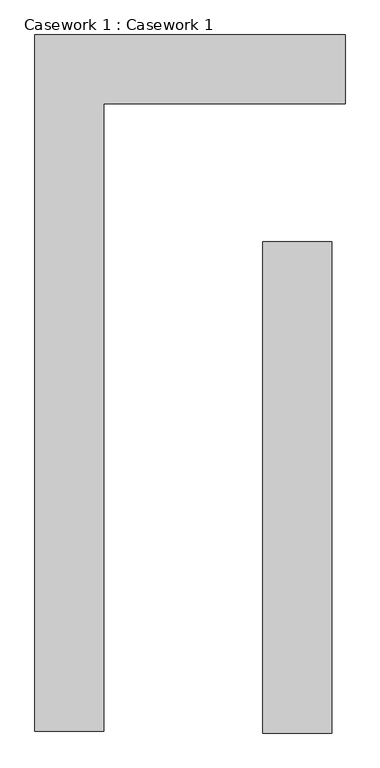
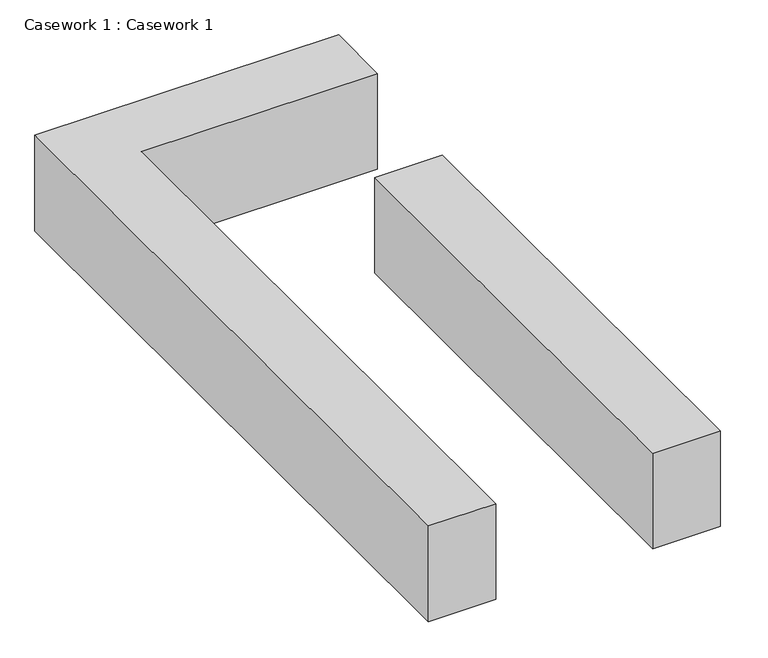
"""IFC4 building model written with IfcOpenShell, lengths in millimetres: furniture geometry, Casework 1 : Casework 1."""

import ifcopenshell
import ifcopenshell.guid

model = None  # the IFC model being written
_history = None  # IfcOwnerHistory: only IFC2X3 demands one
_inside = {}  # id of a spatial element -> (the spatial element, [elements in it])
_under = {}  # id of a project, library or spatial element -> (it, [spatial elements below it])
_declared = {}  # id of a project -> (the project, [libraries it declares])
_typed = {}  # id of a type object -> (the type object, [elements of that type])
_made_of = {}  # id of a material, layer set ... -> (it, [elements and type objects made of it])


def new_model(schema):
    """Start an empty IFC model of exactly this schema.

    Asked for "IFC4X3", IfcOpenShell would pick the latest addendum, in which some entities
    have other attributes; the version numbers below select the first issue.
    IFC2X3 requires an IfcOwnerHistory on every rooted entity: one is made here for all.
    """
    global model, _history
    if schema == "IFC4X3":
        model = ifcopenshell.file(schema_version=(4, 3, 0, 0))
    else:
        model = ifcopenshell.file(schema=schema)
    _inside.clear()
    _under.clear()
    _declared.clear()
    _typed.clear()
    _made_of.clear()
    _history = None
    if model.schema == "IFC2X3":
        org = make("IfcOrganization", Name="unknown")
        user = make(
            "IfcPersonAndOrganization",
            ThePerson=make("IfcPerson", FamilyName="unknown"),
            TheOrganization=org,
        )
        app = make(
            "IfcApplication",
            ApplicationDeveloper=org,
            Version="unknown",
            ApplicationFullName="unknown",
            ApplicationIdentifier="unknown",
        )
        _history = make(
            "IfcOwnerHistory",
            OwningUser=user,
            OwningApplication=app,
            ChangeAction="ADDED",
            CreationDate=0,
        )
    return model


def make(cls, **values):
    """One entity of the class cls with the attributes given. An attribute that is None is left unset."""
    return model.create_entity(
        cls, **{name: value for name, value in values.items() if value is not None}
    )


def rooted(cls, **values):
    """An entity with a GlobalId (a new one), such as an element, a storey or a relation."""
    return make(cls, GlobalId=ifcopenshell.guid.new(), OwnerHistory=_history, **values)


def si_unit(unit_type, name, prefix=None):
    """IfcSIUnit, for example si_unit("LENGTHUNIT", "METRE", prefix="MILLI")."""
    return make("IfcSIUnit", UnitType=unit_type, Prefix=prefix, Name=name)


def assignment(units):
    """IfcUnitAssignment: the units of a project."""
    return None if units is None else make("IfcUnitAssignment", Units=units)


def point(xyz):
    """IfcCartesianPoint."""
    return None if xyz is None else make("IfcCartesianPoint", Coordinates=xyz)


def direction(xyz):
    """IfcDirection."""
    return None if xyz is None else make("IfcDirection", DirectionRatios=xyz)


def frame(location, z_axis=None, x_axis=None):
    """IfcAxis2Placement3D, a coordinate frame: its origin and axes. An axis left out is left unset."""
    return make(
        "IfcAxis2Placement3D",
        Location=point(location),
        Axis=direction(z_axis),
        RefDirection=direction(x_axis),
    )


def origin():
    """The frame at (0, 0, 0) with its axes left unset."""
    return frame((0.0, 0.0, 0.0))


def origin_with_axes():
    """The frame at (0, 0, 0) with the z axis (0, 0, 1) and the x axis (1, 0, 0) written out."""
    return frame((0.0, 0.0, 0.0), z_axis=(0.0, 0.0, 1.0), x_axis=(1.0, 0.0, 0.0))


def place(relative_to, where):
    """IfcLocalPlacement: puts the frame where relative to a parent placement (None: the world)."""
    return make(
        "IfcLocalPlacement", PlacementRelTo=relative_to, RelativePlacement=where
    )


def context(
    kind, dimensions, precision=None, world=None, true_north=None, identifier=None
):
    """IfcGeometricRepresentationContext, for example the 3D "Model" context."""
    return make(
        "IfcGeometricRepresentationContext",
        ContextIdentifier=identifier,
        ContextType=kind,
        CoordinateSpaceDimension=dimensions,
        Precision=precision,
        WorldCoordinateSystem=world,
        TrueNorth=true_north,
    )


def project(units=None, contexts=None):
    """IfcProject with its units and contexts."""
    return rooted(
        "IfcProject",
        Name="project",
        RepresentationContexts=contexts,
        UnitsInContext=assignment(units),
    )


def spatial(cls, under=None, at=None, **own):
    """A site, building, storey or space (cls), placed at a placement, below another one or the project."""
    s = rooted(cls, ObjectPlacement=at, **own)
    if under is not None:
        _under.setdefault(under.id(), (under, []))[1].append(s)
    return s


def polyline(points):
    """IfcPolyline through the points."""
    return make("IfcPolyline", Points=[point(p) for p in points])


def outline(outer, holes=None, kind="AREA"):
    """IfcArbitraryClosedProfileDef: a profile drawn as a closed curve; with holes, ...WithVoids."""
    if holes is None:
        return make("IfcArbitraryClosedProfileDef", ProfileType=kind, OuterCurve=outer)
    return make(
        "IfcArbitraryProfileDefWithVoids",
        ProfileType=kind,
        OuterCurve=outer,
        InnerCurves=holes,
    )


def extrude(swept, where, along, depth):
    """IfcExtrudedAreaSolid: the profile swept, set in the frame where, extruded along a direction by depth."""
    return make(
        "IfcExtrudedAreaSolid",
        SweptArea=swept,
        Position=where,
        ExtrudedDirection=direction(along),
        Depth=depth,
    )


def shape(context_of_items, identifier, shape_type, items):
    """IfcShapeRepresentation: the items that make up one representation, for example the "Body"."""
    return make(
        "IfcShapeRepresentation",
        ContextOfItems=context_of_items,
        RepresentationIdentifier=identifier,
        RepresentationType=shape_type,
        Items=items,
    )


def source(mapping_origin, context_of_items, identifier, shape_type, items):
    """IfcRepresentationMap: a shape defined once, which mapped items show again and again."""
    return make(
        "IfcRepresentationMap",
        MappingOrigin=mapping_origin,
        MappedRepresentation=shape(context_of_items, identifier, shape_type, items),
    )


def transform(
    local_origin,
    x_axis=None,
    y_axis=None,
    z_axis=None,
    scale=None,
    scale2=None,
    scale3=None,
    uniform=True,
):
    """IfcCartesianTransformationOperator3D, or its non-uniform kind. x_axis, y_axis, z_axis: its Axis1, 2, 3."""
    if uniform:
        return make(
            "IfcCartesianTransformationOperator3D",
            Axis1=direction(x_axis),
            Axis2=direction(y_axis),
            LocalOrigin=point(local_origin),
            Scale=scale,
            Axis3=direction(z_axis),
        )
    return make(
        "IfcCartesianTransformationOperator3DnonUniform",
        Axis1=direction(x_axis),
        Axis2=direction(y_axis),
        LocalOrigin=point(local_origin),
        Scale=scale,
        Axis3=direction(z_axis),
        Scale2=scale2,
        Scale3=scale3,
    )


def mapped(mapping_source, mapping_target):
    """IfcMappedItem: shows the shape of a source again, moved by a transform."""
    return make(
        "IfcMappedItem", MappingSource=mapping_source, MappingTarget=mapping_target
    )


def made_of(thing, what):
    """Note that an element or type object is made of a material, layer set ...; save() writes the relation."""
    if what is not None:
        _made_of.setdefault(what.id(), (what, []))[1].append(thing)
    return thing


def element(
    cls,
    number,
    at=None,
    inside=None,
    cuts=None,
    type_object=None,
    material=None,
    context=None,
    identifier="Body",
    shape_type=None,
    held_by="IfcProductDefinitionShape",
    body=None,
    shapes=None,
    **own,
):
    """One element of the class cls, such as IfcWall. Its Tag is "e" and its number.

    at: its placement. inside: the storey or other place that contains it. cuts: it is an
    opening in that element (IfcRelVoidsElement). A single representation is given by context,
    identifier, shape_type and body (its items); several are given by shapes. held_by: the class
    of the entity that holds the representations. save() writes the other relations.
    """
    e = rooted(cls, Tag="e%d" % number, ObjectPlacement=at, **own)
    if body is not None:
        shapes = [shape(context, identifier, shape_type, body)]
    if shapes is not None:
        e.Representation = make(held_by, Representations=shapes)
    if inside is not None:
        _inside.setdefault(inside.id(), (inside, []))[1].append(e)
    if cuts is not None:
        rooted(
            "IfcRelVoidsElement", RelatingBuildingElement=cuts, RelatedOpeningElement=e
        )
    if type_object is not None:
        _typed.setdefault(type_object.id(), (type_object, []))[1].append(e)
    return made_of(e, material)


def aggregate(whole, parts):
    """IfcRelAggregates: a whole, such as a stair, and the parts it consists of."""
    return rooted("IfcRelAggregates", RelatingObject=whole, RelatedObjects=parts)


def save(model, path):
    """Write the relations noted so far, then the file.

    IfcRelAggregates (storeys below a building ...), IfcRelContainedInSpatialStructure (elements
    in a storey), IfcRelDefinesByType, IfcRelAssociatesMaterial and IfcRelDeclares: one each for
    every whole, place, type object, material and project.
    """
    for whole, parts in _under.values():
        aggregate(whole, parts)
    for where, things in _inside.values():
        rooted(
            "IfcRelContainedInSpatialStructure",
            RelatedElements=things,
            RelatingStructure=where,
        )
    for kind, things in _typed.values():
        rooted("IfcRelDefinesByType", RelatedObjects=things, RelatingType=kind)
    for what, things in _made_of.values():
        rooted("IfcRelAssociatesMaterial", RelatedObjects=things, RelatingMaterial=what)
    for by, libraries in _declared.values():
        rooted("IfcRelDeclares", RelatingContext=by, RelatedDefinitions=libraries)
    model.write(path)


def casework_1_casework_1_232e81b5(model_context):
    return source(origin(), model_context, "Body", "SweptSolid", [
        extrude(outline(polyline([(653847.1867239, -574091.7445091), (653847.1867239, -567932.6413841), (656590.3867239, -567932.6413841), (656590.3867239, -568542.2413841), (654456.7867239, -568542.2413841), (654456.7867239, -574091.7445091), (653847.1867239, -574091.7445091)])), origin_with_axes(), (0.0, 0.0, 1.0), 914.4),
        extrude(outline(polyline([(655863.3117239, -574107.6195091), (655863.3117239, -569761.4413841), (656472.9117239, -569761.4413841), (656472.9117239, -574107.6195091), (655863.3117239, -574107.6195091)])), origin_with_axes(), (0.0, 0.0, 1.0), 914.4),
    ])


if __name__ == "__main__":
    model = new_model("IFC4")
    model_context = context("Model", 3, world=origin())
    ifc_project = project(units=[si_unit("LENGTHUNIT", "METRE", prefix="MILLI")], contexts=[model_context])
    site = spatial("IfcSite", under=ifc_project)
    building = spatial("IfcBuilding", under=site)
    placement = place(None, origin())
    casework_1_casework_1_shape = casework_1_casework_1_232e81b5(model_context)
    element("IfcFurniture", 1, ObjectType="Casework 1 : Casework 1", at=placement, inside=building, context=model_context, shape_type="MappedRepresentation", body=[
        mapped(casework_1_casework_1_shape, transform((0.0, 0.0, 0.0), x_axis=(1.0, 0.0, 0.0), y_axis=(0.0, 1.0, 0.0), z_axis=(0.0, 0.0, 1.0))),
    ])
    save(model, "model.ifc")
